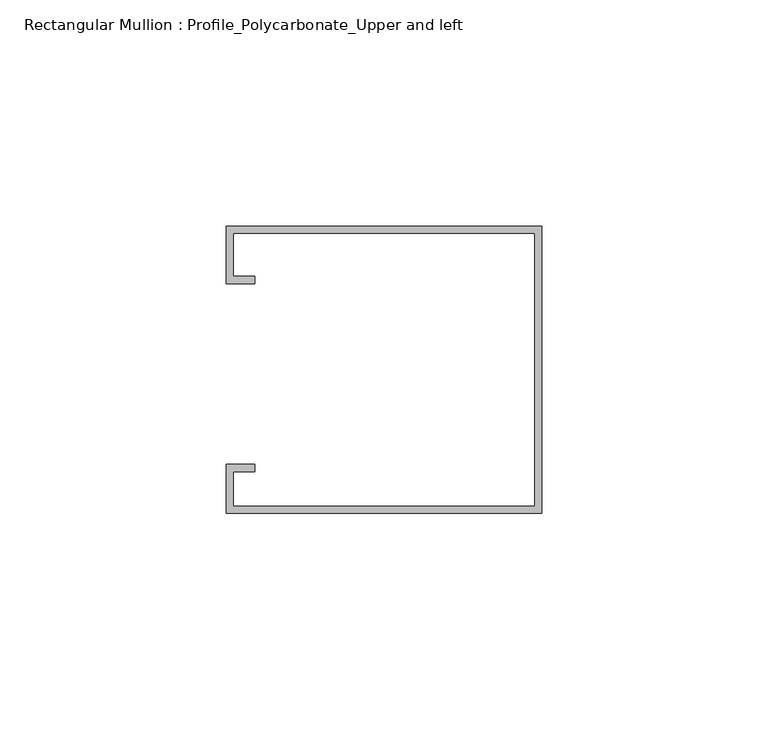
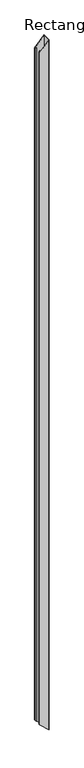
"""IFC4 building model written with IfcOpenShell, lengths in millimetres: member geometry, Rectangular Mullion : Profile_Polycarbonate_Upper and left."""

import ifcopenshell
import ifcopenshell.guid

model = None  # the IFC model being written
_history = None  # IfcOwnerHistory: only IFC2X3 demands one
_inside = {}  # id of a spatial element -> (the spatial element, [elements in it])
_under = {}  # id of a project, library or spatial element -> (it, [spatial elements below it])
_declared = {}  # id of a project -> (the project, [libraries it declares])
_typed = {}  # id of a type object -> (the type object, [elements of that type])
_made_of = {}  # id of a material, layer set ... -> (it, [elements and type objects made of it])


def new_model(schema):
    """Start an empty IFC model of exactly this schema.

    Asked for "IFC4X3", IfcOpenShell would pick the latest addendum, in which some entities
    have other attributes; the version numbers below select the first issue.
    IFC2X3 requires an IfcOwnerHistory on every rooted entity: one is made here for all.
    """
    global model, _history
    if schema == "IFC4X3":
        model = ifcopenshell.file(schema_version=(4, 3, 0, 0))
    else:
        model = ifcopenshell.file(schema=schema)
    _inside.clear()
    _under.clear()
    _declared.clear()
    _typed.clear()
    _made_of.clear()
    _history = None
    if model.schema == "IFC2X3":
        org = make("IfcOrganization", Name="unknown")
        user = make(
            "IfcPersonAndOrganization",
            ThePerson=make("IfcPerson", FamilyName="unknown"),
            TheOrganization=org,
        )
        app = make(
            "IfcApplication",
            ApplicationDeveloper=org,
            Version="unknown",
            ApplicationFullName="unknown",
            ApplicationIdentifier="unknown",
        )
        _history = make(
            "IfcOwnerHistory",
            OwningUser=user,
            OwningApplication=app,
            ChangeAction="ADDED",
            CreationDate=0,
        )
    return model


def make(cls, **values):
    """One entity of the class cls with the attributes given. An attribute that is None is left unset."""
    return model.create_entity(
        cls, **{name: value for name, value in values.items() if value is not None}
    )


def rooted(cls, **values):
    """An entity with a GlobalId (a new one), such as an element, a storey or a relation."""
    return make(cls, GlobalId=ifcopenshell.guid.new(), OwnerHistory=_history, **values)


def si_unit(unit_type, name, prefix=None):
    """IfcSIUnit, for example si_unit("LENGTHUNIT", "METRE", prefix="MILLI")."""
    return make("IfcSIUnit", UnitType=unit_type, Prefix=prefix, Name=name)


def assignment(units):
    """IfcUnitAssignment: the units of a project."""
    return None if units is None else make("IfcUnitAssignment", Units=units)


def point(xyz):
    """IfcCartesianPoint."""
    return None if xyz is None else make("IfcCartesianPoint", Coordinates=xyz)


def direction(xyz):
    """IfcDirection."""
    return None if xyz is None else make("IfcDirection", DirectionRatios=xyz)


def frame(location, z_axis=None, x_axis=None):
    """IfcAxis2Placement3D, a coordinate frame: its origin and axes. An axis left out is left unset."""
    return make(
        "IfcAxis2Placement3D",
        Location=point(location),
        Axis=direction(z_axis),
        RefDirection=direction(x_axis),
    )


def origin():
    """The frame at (0, 0, 0) with its axes left unset."""
    return frame((0.0, 0.0, 0.0))


def place(relative_to, where):
    """IfcLocalPlacement: puts the frame where relative to a parent placement (None: the world)."""
    return make(
        "IfcLocalPlacement", PlacementRelTo=relative_to, RelativePlacement=where
    )


def context(
    kind, dimensions, precision=None, world=None, true_north=None, identifier=None
):
    """IfcGeometricRepresentationContext, for example the 3D "Model" context."""
    return make(
        "IfcGeometricRepresentationContext",
        ContextIdentifier=identifier,
        ContextType=kind,
        CoordinateSpaceDimension=dimensions,
        Precision=precision,
        WorldCoordinateSystem=world,
        TrueNorth=true_north,
    )


def project(units=None, contexts=None):
    """IfcProject with its units and contexts."""
    return rooted(
        "IfcProject",
        Name="project",
        RepresentationContexts=contexts,
        UnitsInContext=assignment(units),
    )


def spatial(cls, under=None, at=None, **own):
    """A site, building, storey or space (cls), placed at a placement, below another one or the project."""
    s = rooted(cls, ObjectPlacement=at, **own)
    if under is not None:
        _under.setdefault(under.id(), (under, []))[1].append(s)
    return s


def faces_of(points, faces, orient=None, outer=None):
    """IfcFace entities. A face is a list of loops; a loop is a list of indices into points, from 0.

    orient and outer hold one flag for each loop. By default every Orientation is true, the
    first loop of a face is its IfcFaceOuterBound and the others are IfcFaceBound.
    """
    made = []
    for i, loops in enumerate(faces):
        bounds = []
        for j, loop in enumerate(loops):
            is_outer = j == 0 if outer is None else outer[i][j]
            bounds.append(
                make(
                    "IfcFaceOuterBound" if is_outer else "IfcFaceBound",
                    Bound=make("IfcPolyLoop", Polygon=[points[k] for k in loop]),
                    Orientation=True if orient is None else orient[i][j],
                )
            )
        made.append(make("IfcFace", Bounds=bounds))
    return made


def faceted_brep(points, faces, orient=None, outer=None, voids=None):
    """IfcFacetedBrep: a solid bounded by flat faces; with voids (closed shells), ...WithVoids."""
    shared = [point(p) for p in points]
    hull = make("IfcClosedShell", CfsFaces=faces_of(shared, faces, orient, outer))
    if voids is None:
        return make("IfcFacetedBrep", Outer=hull)
    return make(
        "IfcFacetedBrepWithVoids",
        Outer=hull,
        Voids=[
            make(cls, CfsFaces=faces_of(shared, fs, o, b)) for cls, fs, o, b in voids
        ],
    )


def shape(context_of_items, identifier, shape_type, items):
    """IfcShapeRepresentation: the items that make up one representation, for example the "Body"."""
    return make(
        "IfcShapeRepresentation",
        ContextOfItems=context_of_items,
        RepresentationIdentifier=identifier,
        RepresentationType=shape_type,
        Items=items,
    )


def source(mapping_origin, context_of_items, identifier, shape_type, items):
    """IfcRepresentationMap: a shape defined once, which mapped items show again and again."""
    return make(
        "IfcRepresentationMap",
        MappingOrigin=mapping_origin,
        MappedRepresentation=shape(context_of_items, identifier, shape_type, items),
    )


def transform(
    local_origin,
    x_axis=None,
    y_axis=None,
    z_axis=None,
    scale=None,
    scale2=None,
    scale3=None,
    uniform=True,
):
    """IfcCartesianTransformationOperator3D, or its non-uniform kind. x_axis, y_axis, z_axis: its Axis1, 2, 3."""
    if uniform:
        return make(
            "IfcCartesianTransformationOperator3D",
            Axis1=direction(x_axis),
            Axis2=direction(y_axis),
            LocalOrigin=point(local_origin),
            Scale=scale,
            Axis3=direction(z_axis),
        )
    return make(
        "IfcCartesianTransformationOperator3DnonUniform",
        Axis1=direction(x_axis),
        Axis2=direction(y_axis),
        LocalOrigin=point(local_origin),
        Scale=scale,
        Axis3=direction(z_axis),
        Scale2=scale2,
        Scale3=scale3,
    )


def mapped(mapping_source, mapping_target):
    """IfcMappedItem: shows the shape of a source again, moved by a transform."""
    return make(
        "IfcMappedItem", MappingSource=mapping_source, MappingTarget=mapping_target
    )


def made_of(thing, what):
    """Note that an element or type object is made of a material, layer set ...; save() writes the relation."""
    if what is not None:
        _made_of.setdefault(what.id(), (what, []))[1].append(thing)
    return thing


def element(
    cls,
    number,
    at=None,
    inside=None,
    cuts=None,
    type_object=None,
    material=None,
    context=None,
    identifier="Body",
    shape_type=None,
    held_by="IfcProductDefinitionShape",
    body=None,
    shapes=None,
    **own,
):
    """One element of the class cls, such as IfcWall. Its Tag is "e" and its number.

    at: its placement. inside: the storey or other place that contains it. cuts: it is an
    opening in that element (IfcRelVoidsElement). A single representation is given by context,
    identifier, shape_type and body (its items); several are given by shapes. held_by: the class
    of the entity that holds the representations. save() writes the other relations.
    """
    e = rooted(cls, Tag="e%d" % number, ObjectPlacement=at, **own)
    if body is not None:
        shapes = [shape(context, identifier, shape_type, body)]
    if shapes is not None:
        e.Representation = make(held_by, Representations=shapes)
    if inside is not None:
        _inside.setdefault(inside.id(), (inside, []))[1].append(e)
    if cuts is not None:
        rooted(
            "IfcRelVoidsElement", RelatingBuildingElement=cuts, RelatedOpeningElement=e
        )
    if type_object is not None:
        _typed.setdefault(type_object.id(), (type_object, []))[1].append(e)
    return made_of(e, material)


def aggregate(whole, parts):
    """IfcRelAggregates: a whole, such as a stair, and the parts it consists of."""
    return rooted("IfcRelAggregates", RelatingObject=whole, RelatedObjects=parts)


def save(model, path):
    """Write the relations noted so far, then the file.

    IfcRelAggregates (storeys below a building ...), IfcRelContainedInSpatialStructure (elements
    in a storey), IfcRelDefinesByType, IfcRelAssociatesMaterial and IfcRelDeclares: one each for
    every whole, place, type object, material and project.
    """
    for whole, parts in _under.values():
        aggregate(whole, parts)
    for where, things in _inside.values():
        rooted(
            "IfcRelContainedInSpatialStructure",
            RelatedElements=things,
            RelatingStructure=where,
        )
    for kind, things in _typed.values():
        rooted("IfcRelDefinesByType", RelatedObjects=things, RelatingType=kind)
    for what, things in _made_of.values():
        rooted("IfcRelAssociatesMaterial", RelatedObjects=things, RelatingMaterial=what)
    for by, libraries in _declared.values():
        rooted("IfcRelDeclares", RelatingContext=by, RelatedDefinitions=libraries)
    model.write(path)


def rectangular_mullion_profile_polycarbonate_upper_and_left_79633bbb(model_context):
    return source(origin(), model_context, "Body", "Brep", [
        faceted_brep([(-69.85, 32.7, -75.9129484), (0.0, 32.7, 0.0), (0.0, 32.7, -5338.1517667), (-69.85, 32.7, -5273.880485), (-69.85, 20.0, -75.9129484), (-69.85, 20.0, -5273.880485), (-63.5, 20.0, -69.0117713), (-63.5, 20.0, -5279.7233287), (-63.5, 21.5875, -69.0117713), (-63.5, 21.5875, -5279.7233287), (-68.2625, 21.5875, -74.1876542), (-68.2625, 21.5875, -5275.3411959), (-68.2625, 31.1125, -74.1876542), (-68.2625, 31.1125, -5275.3411959), (-1.5875, 31.1125, -1.7252943), (-1.5875, 31.1125, -5336.6910558), (-1.5875, -29.2125, -1.7252943), (-1.5875, -29.2125, -5336.6910558), (-68.2625, -29.2125, -74.1876542), (-68.2625, -29.2125, -5275.3411959), (-68.2625, -21.5875, -74.1876542), (-68.2625, -21.5875, -5275.3411959), (-63.5, -21.5875, -69.0117713), (-63.5, -21.5875, -5279.7233287), (-63.5, -20.0, -69.0117713), (-63.5, -20.0, -5279.7233287), (-69.85, -20.0, -75.9129484), (-69.85, -20.0, -5273.880485), (-69.85, -30.8, -75.9129484), (-69.85, -30.8, -5273.880485), (0.0, -30.8, 0.0), (0.0, -30.8, -5338.1517667)], [[[0, 1, 2, 3]], [[4, 0, 3, 5]], [[6, 4, 5, 7]], [[8, 6, 7, 9]], [[10, 8, 9, 11]], [[12, 10, 11, 13]], [[14, 12, 13, 15]], [[16, 14, 15, 17]], [[18, 16, 17, 19]], [[20, 18, 19, 21]], [[22, 20, 21, 23]], [[24, 22, 23, 25]], [[26, 24, 25, 27]], [[28, 26, 27, 29]], [[30, 28, 29, 31]], [[1, 30, 31, 2]], [[1, 0, 4, 6, 8, 10, 12, 14, 16, 18, 20, 22, 24, 26, 28, 30]], [[2, 31, 29, 27, 25, 23, 21, 19, 17, 15, 13, 11, 9, 7, 5, 3]]]),
    ])


if __name__ == "__main__":
    model = new_model("IFC4")
    model_context = context("Model", 3, world=origin())
    ifc_project = project(units=[si_unit("LENGTHUNIT", "METRE", prefix="MILLI")], contexts=[model_context])
    site = spatial("IfcSite", under=ifc_project)
    building = spatial("IfcBuilding", under=site)
    placement = place(None, origin())
    rectangular_mullion_profile_polycarbonate_upper_and_left_shape = rectangular_mullion_profile_polycarbonate_upper_and_left_79633bbb(model_context)
    element("IfcMember", 1, ObjectType="Rectangular Mullion : Profile_Polycarbonate_Upper and left", at=placement, inside=building, context=model_context, shape_type="MappedRepresentation", body=[
        mapped(rectangular_mullion_profile_polycarbonate_upper_and_left_shape, transform((0.0, 0.0, 0.0), x_axis=(1.0, 0.0, 0.0), y_axis=(0.0, 1.0, 0.0), z_axis=(0.0, 0.0, 1.0))),
    ])
    save(model, "model.ifc")

# Revit data of these elements
# Type "Rectangular Mullion : Profile_Polycarbonate_Upper and left"
#   built-in parameter 1007322 = 0.208333 (stored number, unit not read)
#   built-in parameter 1007321 = 0.00520833 (stored number, unit not read)
#   built-in parameter 1007320 = 0 (stored number, unit not read)
# Element 1 (IfcMember, "Rectangular Mullion : Profile_Polycarbonate_Upper and left")
#   Materials on its faces: "ALUMINUM PROFILE AT POLYCARBONATE PANEL"
# Materials
#   "ALUMINUM PROFILE AT POLYCARBONATE PANEL": class "Metal", colour RGB 244 244 244, transparency 0, Description = "Aluminum 6061", Cost = 0
